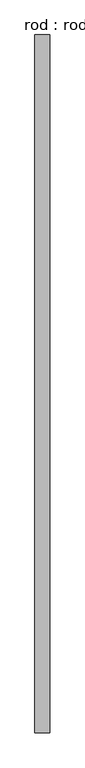
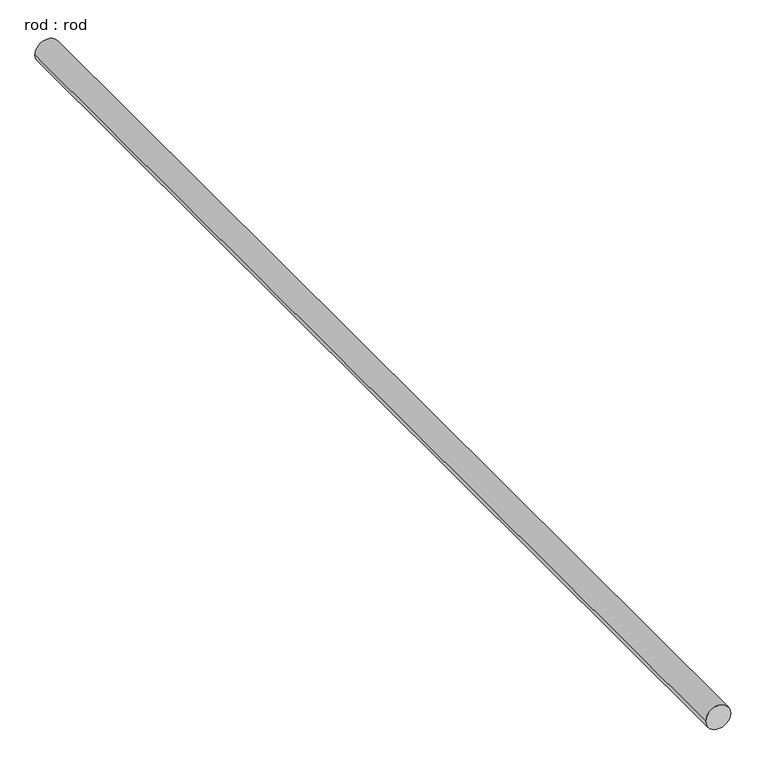
"""IFC4 building model written with IfcOpenShell, lengths in millimetres: proxy geometry, rod : rod."""

from ifc_helpers import new_model, si_unit, point, frame, frame_2d, origin, place, context, project, spatial, circle_curve, trimmed, segment, composite_curve, outline, extrude, source, transform, mapped, element, save


def rod_rod_194314e7(model_context):
    return source(origin(), model_context, "Body", "SweptSolid", [
        extrude(outline(composite_curve([segment(trimmed(circle_curve(frame_2d((0.0108462, 0.0)), 200.0), [point((0.0108462, 200.0))], [point((0.0108462, -200.0))], False, "CARTESIAN"), True, "CONTINUOUS"), segment(trimmed(circle_curve(frame_2d((0.0108462, 0.0)), 200.0), [point((0.0108462, -200.0))], [point((0.0108462, 200.0))], False, "CARTESIAN"), True, "CONTINUOUS")], self_intersect=False)), frame((0.0, -5265.5995607, 0.0), z_axis=(0.0, 1.0, 0.0), x_axis=(0.0, 0.0, 1.0)), (0.0, 0.0, 1.0), 18716.656352),
    ])


if __name__ == "__main__":
    model = new_model("IFC4")
    model_context = context("Model", 3, world=origin())
    ifc_project = project(units=[si_unit("LENGTHUNIT", "METRE", prefix="MILLI")], contexts=[model_context])
    site = spatial("IfcSite", under=ifc_project)
    building = spatial("IfcBuilding", under=site)
    placement = place(None, origin())
    rod_rod_shape = rod_rod_194314e7(model_context)
    element("IfcBuildingElementProxy", 1, Name="rod : rod", ObjectType="rod : rod", at=placement, inside=building, context=model_context, shape_type="MappedRepresentation", body=[
        mapped(rod_rod_shape, transform((0.0, 0.0, 0.0), x_axis=(1.0, 0.0, 0.0), y_axis=(0.0, 1.0, 0.0), z_axis=(0.0, 0.0, 1.0))),
    ])
    save(model, "model.ifc")

# Revit data of these elements
# Type "rod : rod"
#   Default Elevation = 0
